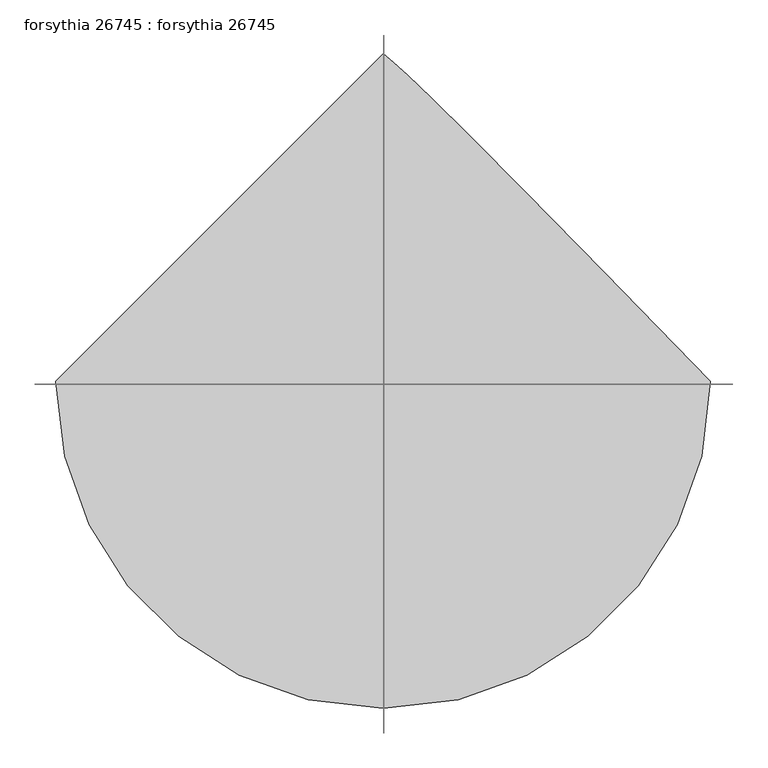
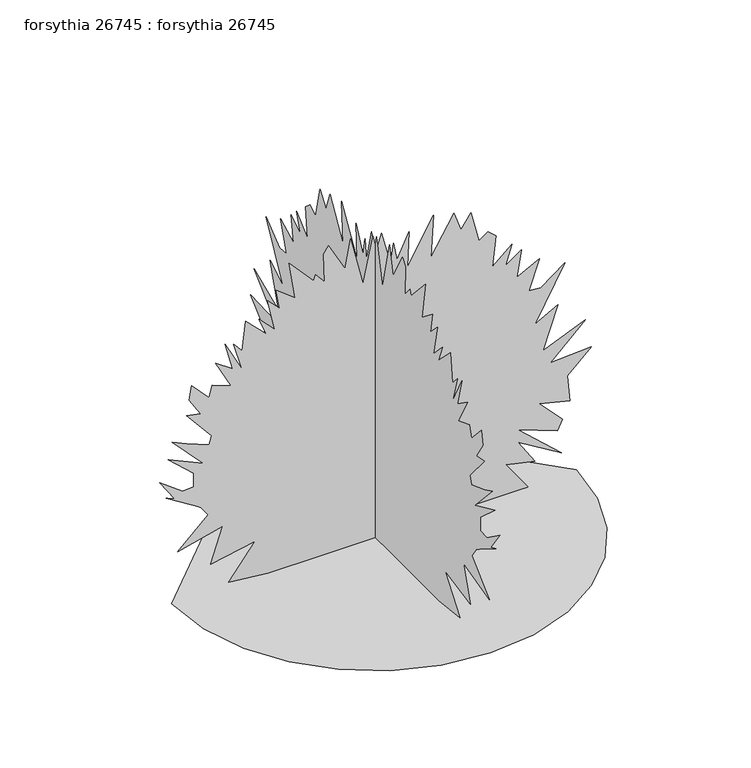
"""IFC4 building model written with IfcOpenShell, lengths in millimetres: proxy geometry, forsythia 26745 : forsythia 26745."""

import ifcopenshell
import ifcopenshell.guid

model = None  # the IFC model being written
_history = None  # IfcOwnerHistory: only IFC2X3 demands one
_inside = {}  # id of a spatial element -> (the spatial element, [elements in it])
_under = {}  # id of a project, library or spatial element -> (it, [spatial elements below it])
_declared = {}  # id of a project -> (the project, [libraries it declares])
_typed = {}  # id of a type object -> (the type object, [elements of that type])
_made_of = {}  # id of a material, layer set ... -> (it, [elements and type objects made of it])


def new_model(schema):
    """Start an empty IFC model of exactly this schema.

    Asked for "IFC4X3", IfcOpenShell would pick the latest addendum, in which some entities
    have other attributes; the version numbers below select the first issue.
    IFC2X3 requires an IfcOwnerHistory on every rooted entity: one is made here for all.
    """
    global model, _history
    if schema == "IFC4X3":
        model = ifcopenshell.file(schema_version=(4, 3, 0, 0))
    else:
        model = ifcopenshell.file(schema=schema)
    _inside.clear()
    _under.clear()
    _declared.clear()
    _typed.clear()
    _made_of.clear()
    _history = None
    if model.schema == "IFC2X3":
        org = make("IfcOrganization", Name="unknown")
        user = make(
            "IfcPersonAndOrganization",
            ThePerson=make("IfcPerson", FamilyName="unknown"),
            TheOrganization=org,
        )
        app = make(
            "IfcApplication",
            ApplicationDeveloper=org,
            Version="unknown",
            ApplicationFullName="unknown",
            ApplicationIdentifier="unknown",
        )
        _history = make(
            "IfcOwnerHistory",
            OwningUser=user,
            OwningApplication=app,
            ChangeAction="ADDED",
            CreationDate=0,
        )
    return model


def make(cls, **values):
    """One entity of the class cls with the attributes given. An attribute that is None is left unset."""
    return model.create_entity(
        cls, **{name: value for name, value in values.items() if value is not None}
    )


def rooted(cls, **values):
    """An entity with a GlobalId (a new one), such as an element, a storey or a relation."""
    return make(cls, GlobalId=ifcopenshell.guid.new(), OwnerHistory=_history, **values)


def si_unit(unit_type, name, prefix=None):
    """IfcSIUnit, for example si_unit("LENGTHUNIT", "METRE", prefix="MILLI")."""
    return make("IfcSIUnit", UnitType=unit_type, Prefix=prefix, Name=name)


def assignment(units):
    """IfcUnitAssignment: the units of a project."""
    return None if units is None else make("IfcUnitAssignment", Units=units)


def point(xyz):
    """IfcCartesianPoint."""
    return None if xyz is None else make("IfcCartesianPoint", Coordinates=xyz)


def direction(xyz):
    """IfcDirection."""
    return None if xyz is None else make("IfcDirection", DirectionRatios=xyz)


def frame(location, z_axis=None, x_axis=None):
    """IfcAxis2Placement3D, a coordinate frame: its origin and axes. An axis left out is left unset."""
    return make(
        "IfcAxis2Placement3D",
        Location=point(location),
        Axis=direction(z_axis),
        RefDirection=direction(x_axis),
    )


def origin():
    """The frame at (0, 0, 0) with its axes left unset."""
    return frame((0.0, 0.0, 0.0))


def place(relative_to, where):
    """IfcLocalPlacement: puts the frame where relative to a parent placement (None: the world)."""
    return make(
        "IfcLocalPlacement", PlacementRelTo=relative_to, RelativePlacement=where
    )


def context(
    kind, dimensions, precision=None, world=None, true_north=None, identifier=None
):
    """IfcGeometricRepresentationContext, for example the 3D "Model" context."""
    return make(
        "IfcGeometricRepresentationContext",
        ContextIdentifier=identifier,
        ContextType=kind,
        CoordinateSpaceDimension=dimensions,
        Precision=precision,
        WorldCoordinateSystem=world,
        TrueNorth=true_north,
    )


def project(units=None, contexts=None):
    """IfcProject with its units and contexts."""
    return rooted(
        "IfcProject",
        Name="project",
        RepresentationContexts=contexts,
        UnitsInContext=assignment(units),
    )


def spatial(cls, under=None, at=None, **own):
    """A site, building, storey or space (cls), placed at a placement, below another one or the project."""
    s = rooted(cls, ObjectPlacement=at, **own)
    if under is not None:
        _under.setdefault(under.id(), (under, []))[1].append(s)
    return s


def point_list(points):
    """IfcCartesianPointList2D or 3D."""
    cls = (
        "IfcCartesianPointList2D" if len(points[0]) == 2 else "IfcCartesianPointList3D"
    )
    return make(cls, CoordList=points)


def triangles(points, corners, closed=None, point_numbers=None):
    """IfcTriangulatedFaceSet: each triangle names its three corners, points numbered from 1."""
    return make(
        "IfcTriangulatedFaceSet",
        Coordinates=point_list(points),
        Closed=closed,
        CoordIndex=corners,
        PnIndex=point_numbers,
    )


def shape(context_of_items, identifier, shape_type, items):
    """IfcShapeRepresentation: the items that make up one representation, for example the "Body"."""
    return make(
        "IfcShapeRepresentation",
        ContextOfItems=context_of_items,
        RepresentationIdentifier=identifier,
        RepresentationType=shape_type,
        Items=items,
    )


def source(mapping_origin, context_of_items, identifier, shape_type, items):
    """IfcRepresentationMap: a shape defined once, which mapped items show again and again."""
    return make(
        "IfcRepresentationMap",
        MappingOrigin=mapping_origin,
        MappedRepresentation=shape(context_of_items, identifier, shape_type, items),
    )


def transform(
    local_origin,
    x_axis=None,
    y_axis=None,
    z_axis=None,
    scale=None,
    scale2=None,
    scale3=None,
    uniform=True,
):
    """IfcCartesianTransformationOperator3D, or its non-uniform kind. x_axis, y_axis, z_axis: its Axis1, 2, 3."""
    if uniform:
        return make(
            "IfcCartesianTransformationOperator3D",
            Axis1=direction(x_axis),
            Axis2=direction(y_axis),
            LocalOrigin=point(local_origin),
            Scale=scale,
            Axis3=direction(z_axis),
        )
    return make(
        "IfcCartesianTransformationOperator3DnonUniform",
        Axis1=direction(x_axis),
        Axis2=direction(y_axis),
        LocalOrigin=point(local_origin),
        Scale=scale,
        Axis3=direction(z_axis),
        Scale2=scale2,
        Scale3=scale3,
    )


def mapped(mapping_source, mapping_target):
    """IfcMappedItem: shows the shape of a source again, moved by a transform."""
    return make(
        "IfcMappedItem", MappingSource=mapping_source, MappingTarget=mapping_target
    )


def made_of(thing, what):
    """Note that an element or type object is made of a material, layer set ...; save() writes the relation."""
    if what is not None:
        _made_of.setdefault(what.id(), (what, []))[1].append(thing)
    return thing


def element(
    cls,
    number,
    at=None,
    inside=None,
    cuts=None,
    type_object=None,
    material=None,
    context=None,
    identifier="Body",
    shape_type=None,
    held_by="IfcProductDefinitionShape",
    body=None,
    shapes=None,
    **own,
):
    """One element of the class cls, such as IfcWall. Its Tag is "e" and its number.

    at: its placement. inside: the storey or other place that contains it. cuts: it is an
    opening in that element (IfcRelVoidsElement). A single representation is given by context,
    identifier, shape_type and body (its items); several are given by shapes. held_by: the class
    of the entity that holds the representations. save() writes the other relations.
    """
    e = rooted(cls, Tag="e%d" % number, ObjectPlacement=at, **own)
    if body is not None:
        shapes = [shape(context, identifier, shape_type, body)]
    if shapes is not None:
        e.Representation = make(held_by, Representations=shapes)
    if inside is not None:
        _inside.setdefault(inside.id(), (inside, []))[1].append(e)
    if cuts is not None:
        rooted(
            "IfcRelVoidsElement", RelatingBuildingElement=cuts, RelatedOpeningElement=e
        )
    if type_object is not None:
        _typed.setdefault(type_object.id(), (type_object, []))[1].append(e)
    return made_of(e, material)


def aggregate(whole, parts):
    """IfcRelAggregates: a whole, such as a stair, and the parts it consists of."""
    return rooted("IfcRelAggregates", RelatingObject=whole, RelatedObjects=parts)


def save(model, path):
    """Write the relations noted so far, then the file.

    IfcRelAggregates (storeys below a building ...), IfcRelContainedInSpatialStructure (elements
    in a storey), IfcRelDefinesByType, IfcRelAssociatesMaterial and IfcRelDeclares: one each for
    every whole, place, type object, material and project.
    """
    for whole, parts in _under.values():
        aggregate(whole, parts)
    for where, things in _inside.values():
        rooted(
            "IfcRelContainedInSpatialStructure",
            RelatedElements=things,
            RelatingStructure=where,
        )
    for kind, things in _typed.values():
        rooted("IfcRelDefinesByType", RelatedObjects=things, RelatingType=kind)
    for what, things in _made_of.values():
        rooted("IfcRelAssociatesMaterial", RelatedObjects=things, RelatingMaterial=what)
    for by, libraries in _declared.values():
        rooted("IfcRelDeclares", RelatingContext=by, RelatedDefinitions=libraries)
    model.write(path)


def forsythia_26745_forsythia_26745_3ae10d36(model_context):
    return source(origin(), model_context, "Body", "Tessellation", [
        triangles([(-1519.5040535, 0.0, 0.0002833), (-1479.3336857, -348.1690825, 0.0002833), (-1364.9291862, -667.9078508, 0.0002833), (-1185.447191, -950.0545097, 0.0002833), (-950.0545097, -1185.447191, 0.0002833), (-667.9078508, -1364.9291862, 0.0002833), (-348.1690825, -1479.3336857, 0.0002833), (6.64e-05, -1519.5040535, 0.0002833), (348.1690825, -1479.3336857, 0.0002833), (667.9078508, -1364.9291862, 0.0002833), (950.0545097, -1185.447191, 0.0002833), (1185.447191, -950.0545097, 0.0002833), (1364.9291862, -667.9078508, 0.0002833), (1479.3336857, -348.1690825, 0.0002833), (1519.5040535, 0.0001328, 0.0002833), (1025.698439, 506.5233338, 0.0002833), (659.6172232, 879.4549673, 0.0002833), (399.9699903, 1141.05804, 0.0002833), (225.4722113, 1313.5981625, 0.0002833), (114.8360501, 1419.3438881, 0.0002833), (46.774248, 1480.5555588, 0.0002833), (-0.0001993, 1519.5040535, 0.0002833), (-792.3428427, -13.4822871, 0.037948), (-1099.2418425, -13.4822621, 31.9687972), (-901.0348274, -13.4822871, 287.7194292), (-1233.5117718, -13.4822871, 223.7813261), (-1143.9993576, -13.4822871, 492.3196223), (-1482.8669003, -13.4822871, 409.2003862), (-1252.691415, -13.482312, 620.1937574), (-1310.2352863, -13.482312, 703.3130299), (-1565.9861, -13.482312, 863.1557442), (-1502.0490143, -13.482312, 837.5804157), (-1617.1342861, -13.482312, 1003.8188152), (-1444.505143, -13.482312, 875.9446438), (-1361.3859432, -13.482312, 882.3378582), (-1361.3859432, -13.482312, 991.0299156), (-1553.1972004, -13.4823382, 1163.6615295), (-1291.0531723, -13.4823382, 1042.1805725), (-1521.2286575, -13.4823382, 1291.5383171), (-1412.5366001, -13.4823382, 1240.3875149), (-1246.2982006, -13.4823382, 1176.4505018), (-1227.1160866, -13.4823382, 1240.3875149), (-1412.5366001, -13.4823382, 1464.1673149), (-1310.2352863, -13.4823382, 1444.987817), (-1393.3544861, -13.4823631, 1579.2552029), (-1374.1723721, -13.4823631, 1687.9497311), (-1246.2982006, -13.4823631, 1547.28666), (-1220.7228722, -13.4823631, 1636.7990742), (-1080.0597284, -13.4823631, 1585.6482719), (-1195.147471, -13.4823631, 1803.0374737), (-1067.2732996, -13.4823631, 1713.5250595), (-1124.8171709, -13.4823881, 1930.9116451), (-996.9429995, -13.4823631, 1687.9497311), (-1060.8800852, -13.4823881, 1905.3363167), (-996.9429995, -13.4823631, 1835.0060165), (-971.367671, -13.4823881, 2058.7858166), (-817.9181711, -13.4823881, 1905.3363167), (-869.0663572, -13.4823881, 2039.6061733), (-753.9785419, -13.4823881, 1918.1252163), (-805.1292715, -13.4823881, 2161.0871304), (-715.6167847, -13.4823881, 2071.5747162), (-741.1921858, -13.4823881, 2225.0242161), (-600.5290421, -13.4823881, 2116.3296879), (-645.2865572, -13.4824142, 2404.0490444), (-459.8659347, -13.4823881, 2199.4488876), (-447.0795422, -13.4823881, 2244.2063301), (-379.2689283, -13.4823881, 2162.8804802), (-385.6646862, -13.4824142, 2386.6602802), (-347.290248, -13.4824142, 2438.4078484), (-223.176294, -13.4824142, 2213.9981449), (-182.9654127, -13.4823631, 2435.1743248), (-90.8322191, -13.4823631, 2047.6376598), (-12.3045871, -13.4824142, 2397.6559753), (13.2704245, -13.4823881, 2276.174873), (51.6330312, -13.4824142, 2397.6559753), (115.5706256, -13.4823881, 2135.5118019), (141.1454544, -13.4823881, 2288.9613018), (166.7205467, -13.4823881, 2148.2982307), (256.2334877, -13.4824142, 2340.1119587), (243.445551, -13.4823881, 2065.1815018), (441.6515305, -13.4824142, 2404.0490444), (422.4693801, -13.4823881, 2077.9679306), (595.1010303, -13.4824142, 2365.6874325), (646.2517599, -13.4823881, 2218.6310017), (722.9777452, -13.4824142, 2327.3230591), (780.5216166, -13.4823881, 2084.361145), (850.8519167, -13.4823881, 2129.1185875), (908.395788, -13.4823881, 2077.9679306), (882.8204596, -13.4823631, 1841.399231), (1029.876745, -13.4823881, 1969.2734024), (978.7260881, -13.4823631, 1815.8239025), (1100.2070452, -13.4823881, 1898.9431023), (1068.2385023, -13.4823631, 1694.3429455), (1234.4769745, -13.4823631, 1783.8553596), (1157.7509165, -13.4823631, 1553.6797291), (1247.2634033, -13.4823631, 1547.28666), (1426.2882317, -13.4823631, 1681.5565166), (1202.5084316, -13.4823382, 1272.3560577), (1375.1400455, -13.4823382, 1368.2616863), (1260.0523029, -13.4823382, 1042.1805725), (1579.7377316, -13.4823382, 1176.4505018), (1317.5961742, -13.482312, 927.0928299), (1624.495174, -13.482312, 946.2749439), (1445.4703457, -13.482312, 780.0364717), (1464.6524597, -13.4822871, 575.436315), (1234.4769745, -13.482312, 632.9801863), (1407.1085884, -13.4822871, 447.5621435), (1368.7443604, -13.4822871, 370.838629), (1074.6317167, -13.4822871, 479.5306864), (1400.7129032, -13.4822871, 185.418824), (1074.6317167, -13.4822871, 383.6250578), (1202.5084316, -13.4822871, 185.418824), (985.1193026, -13.4822871, 236.568736), (1151.4898161, -13.4822871, 0.0386752), (19.664159, -13.4822621, 0.0001234), (3.6800653, -809.5031324, 0.0378489), (3.68004, -1116.4046757, 31.9687972), (3.6800653, -918.1977333, 287.7194292), (3.6800653, -1250.6720615, 223.7813261), (3.6800653, -1161.1596474, 492.3196223), (3.6800653, -1500.0298061, 409.2003862), (3.6800653, -1269.8541756, 620.1937574), (3.6800653, -1327.3980469, 703.3130299), (3.6800908, -1583.1463898, 863.1557442), (3.6800908, -1519.209304, 837.5804157), (3.6800908, -1634.2970467, 1003.8188152), (3.6800908, -1461.6654327, 875.9446438), (3.6800908, -1378.5487038, 882.3378582), (3.6800908, -1378.5487038, 991.0299156), (3.6800908, -1570.3599609, 1163.6615295), (3.6800908, -1308.2159328, 1042.1805725), (3.6800908, -1538.3914181, 1291.5383171), (3.6800908, -1429.6968899, 1240.3875149), (3.6800908, -1263.4609612, 1176.4505018), (3.6800908, -1244.2788471, 1240.3875149), (3.6800908, -1429.6968899, 1464.1673149), (3.6800908, -1327.3980469, 1444.987817), (3.6800908, -1410.5172466, 1579.2552029), (3.6801161, -1391.3351326, 1687.9497311), (3.6800908, -1263.4609612, 1547.28666), (3.6800908, -1237.8856327, 1636.7990742), (3.6800908, -1097.2225616, 1585.6508881), (3.6801161, -1212.3103043, 1803.0374737), (3.6800908, -1084.4361328, 1713.5250595), (3.6801161, -1141.9800041, 1930.9116451), (3.6800908, -1014.1032892, 1687.9497311), (3.6801161, -1078.0403749, 1905.3363167), (3.6800908, -1014.1032892, 1835.0060165), (3.6801161, -988.5305042, 2058.7858166), (3.6800908, -835.0784609, 1905.3363167), (3.6801161, -886.2291904, 2039.6061733), (3.6800908, -771.1413752, 1918.1252163), (3.6801161, -822.2921047, 2161.0871304), (3.6801161, -732.7796179, 2071.5747162), (3.6801161, -758.355019, 2225.0242161), (3.6801161, -617.6918753, 2116.3296879), (3.6801161, -662.446847, 2404.0490444), (3.6801161, -477.0287679, 2199.4488876), (3.6801161, -464.2423754, 2244.2063301), (3.6801161, -396.4317616, 2162.8804802), (3.6801161, -402.824976, 2386.6602802), (3.6801161, -364.4530812, 2438.4078484), (3.6801161, -240.3386185, 2213.9981449), (3.6800653, -200.1277554, 2435.1743248), (3.6800653, -107.994798, 2047.640276), (3.6801161, -29.4668878, 2397.6559753), (3.6800908, -3.8919275, 2276.174873), (3.6801161, 34.4707044, 2397.6559753), (3.6800908, 98.408301, 2135.5118019), (3.6800908, 123.9831299, 2288.9613018), (3.6800908, 149.5579678, 2148.3008469), (3.6800908, 239.0706363, 2340.1119587), (3.6800908, 226.2832264, 2065.1815018), (3.6800908, 424.4886972, 2404.0490444), (3.6800908, 405.3090903, 2077.9679306), (3.6800908, 577.9381971, 2365.6874325), (3.6800908, 629.0889267, 2218.6310017), (3.6800908, 705.814912, 2327.3256752), (3.6800908, 763.3587833, 2084.361145), (3.6800908, 833.6890835, 2129.1185875), (3.6800908, 891.2329548, 2077.9679306), (3.6800653, 865.6576263, 1841.399231), (3.6800653, 1012.7139118, 1969.2734024), (3.6800653, 961.5632549, 1815.8239025), (3.6800653, 1083.044212, 1898.9431023), (3.6800653, 1051.0756691, 1694.3429455), (3.6800653, 1217.3141413, 1783.8553596), (3.6800653, 1140.5880833, 1553.6797291), (3.6800653, 1230.1004974, 1547.28666), (3.6800653, 1409.1253258, 1681.5565166), (3.6800653, 1185.3455984, 1272.3560577), (3.6800653, 1357.977285, 1368.2616863), (3.68004, 1242.8895424, 1042.1805725), (3.68004, 1562.5774418, 1176.4505018), (3.68004, 1300.4334137, 927.0928299), (3.68004, 1607.3324135, 946.2749439), (3.68004, 1428.3075851, 780.0364717), (3.68004, 1447.4896992, 575.436315), (3.68004, 1217.3141413, 632.9801863), (3.6800145, 1389.9458279, 447.5621435), (3.6800145, 1351.5840706, 370.838629), (3.68004, 1057.471427, 479.5306864), (3.6800145, 1383.5526134, 185.4185696), (3.68004, 1057.471427, 383.6250578), (3.6800145, 1185.3455984, 185.4185696), (3.6800145, 967.9590128, 236.568736), (3.68004, 1134.3269829, 0.038518), (3.68004, 2.5017556, 0.0)], [[21, 22, 1], [20, 21, 1], [19, 20, 1], [18, 19, 1], [17, 18, 1], [17, 1, 2], [17, 2, 3], [17, 3, 4], [16, 17, 4], [16, 4, 5], [16, 5, 6], [16, 6, 7], [16, 7, 8], [16, 8, 9], [16, 9, 10], [16, 10, 11], [16, 11, 12], [15, 16, 12], [14, 15, 12], [13, 14, 12], [30, 31, 32], [109, 110, 111], [51, 52, 53], [36, 37, 38], [32, 33, 34], [76, 77, 78], [100, 101, 102], [38, 39, 40], [78, 79, 80], [57, 58, 59], [70, 71, 72], [96, 97, 98], [72, 73, 74], [53, 54, 55], [80, 81, 82], [49, 50, 51], [27, 28, 29], [89, 90, 91], [74, 75, 76], [59, 60, 61], [63, 64, 65], [38, 40, 41], [102, 103, 104], [42, 43, 44], [98, 99, 100], [61, 62, 63], [93, 94, 95], [111, 112, 113], [91, 92, 93], [84, 85, 86], [82, 83, 84], [55, 56, 57], [45, 46, 47], [44, 45, 47], [113, 114, 115], [65, 66, 67], [23, 24, 25], [72, 74, 76], [25, 26, 27], [68, 69, 70], [67, 68, 70], [30, 32, 34], [30, 34, 35], [104, 105, 106], [49, 51, 53], [102, 104, 106], [95, 96, 98], [47, 48, 49], [107, 108, 109], [106, 107, 109], [82, 84, 86], [86, 87, 88], [86, 88, 89], [67, 70, 72], [115, 23, 25], [53, 55, 57], [82, 86, 89], [76, 78, 80], [63, 65, 67], [59, 61, 63], [42, 44, 47], [42, 47, 49], [35, 36, 38], [72, 76, 80], [111, 113, 115], [109, 111, 115], [100, 102, 106], [100, 106, 109], [100, 109, 115], [98, 100, 115], [98, 115, 25], [95, 98, 25], [93, 95, 25], [91, 93, 25], [89, 91, 25], [82, 89, 25], [80, 82, 25], [72, 80, 25], [72, 25, 27], [72, 27, 29], [67, 72, 29], [63, 67, 29], [59, 63, 29], [59, 29, 30], [59, 30, 35], [59, 35, 38], [59, 38, 41], [59, 41, 42], [59, 42, 49], [59, 49, 53], [59, 53, 57], [123, 124, 125], [202, 203, 204], [144, 145, 146], [129, 130, 131], [125, 126, 127], [169, 170, 171], [193, 194, 195], [131, 132, 133], [171, 172, 173], [150, 151, 152], [163, 164, 165], [189, 190, 191], [165, 166, 167], [146, 147, 148], [173, 174, 175], [142, 143, 144], [120, 121, 122], [182, 183, 184], [167, 168, 169], [152, 153, 154], [156, 157, 158], [131, 133, 134], [195, 196, 197], [135, 136, 137], [191, 192, 193], [154, 155, 156], [186, 187, 188], [204, 205, 206], [184, 185, 186], [177, 178, 179], [175, 176, 177], [148, 149, 150], [138, 139, 140], [137, 138, 140], [206, 207, 208], [158, 159, 160], [116, 117, 118], [165, 167, 169], [118, 119, 120], [161, 162, 163], [160, 161, 163], [123, 125, 127], [123, 127, 128], [197, 198, 199], [142, 144, 146], [195, 197, 199], [188, 189, 191], [140, 141, 142], [200, 201, 202], [199, 200, 202], [175, 177, 179], [179, 180, 181], [179, 181, 182], [160, 163, 165], [208, 116, 118], [146, 148, 150], [175, 179, 182], [169, 171, 173], [156, 158, 160], [152, 154, 156], [135, 137, 140], [135, 140, 142], [128, 129, 131], [165, 169, 173], [204, 206, 208], [202, 204, 208], [193, 195, 199], [193, 199, 202], [193, 202, 208], [191, 193, 208], [191, 208, 118], [188, 191, 118], [186, 188, 118], [184, 186, 118], [182, 184, 118], [175, 182, 118], [173, 175, 118], [165, 173, 118], [165, 118, 120], [165, 120, 122], [160, 165, 122], [156, 160, 122], [152, 156, 122], [152, 122, 123], [152, 123, 128], [152, 128, 131], [152, 131, 134], [152, 134, 135], [152, 135, 142], [152, 142, 146], [152, 146, 150]], closed=False),
    ])


if __name__ == "__main__":
    model = new_model("IFC4")
    model_context = context("Model", 3, world=origin())
    ifc_project = project(units=[si_unit("LENGTHUNIT", "METRE", prefix="MILLI")], contexts=[model_context])
    site = spatial("IfcSite", under=ifc_project)
    building = spatial("IfcBuilding", under=site)
    placement = place(None, origin())
    forsythia_26745_forsythia_26745_shape = forsythia_26745_forsythia_26745_3ae10d36(model_context)
    element("IfcBuildingElementProxy", 1, Name="forsythia 26745 : forsythia 26745", ObjectType="forsythia 26745 : forsythia 26745", at=placement, inside=building, context=model_context, shape_type="MappedRepresentation", body=[
        mapped(forsythia_26745_forsythia_26745_shape, transform((0.0, 0.0, 0.0), x_axis=(1.0, 0.0, 0.0), y_axis=(0.0, 1.0, 0.0), z_axis=(0.0, 0.0, 1.0))),
    ])
    save(model, "model.ifc")

# Revit data of these elements
# Type "forsythia 26745 : forsythia 26745"
#   built-in parameter 1005195 = "RPC-16-G2F6-877X-GLVN-N000-ST1L-LVER-AU"
#   Height = 0
